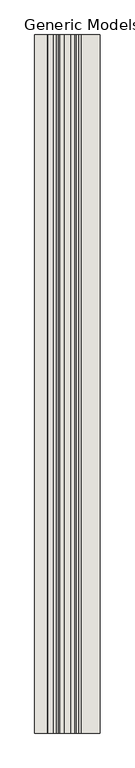
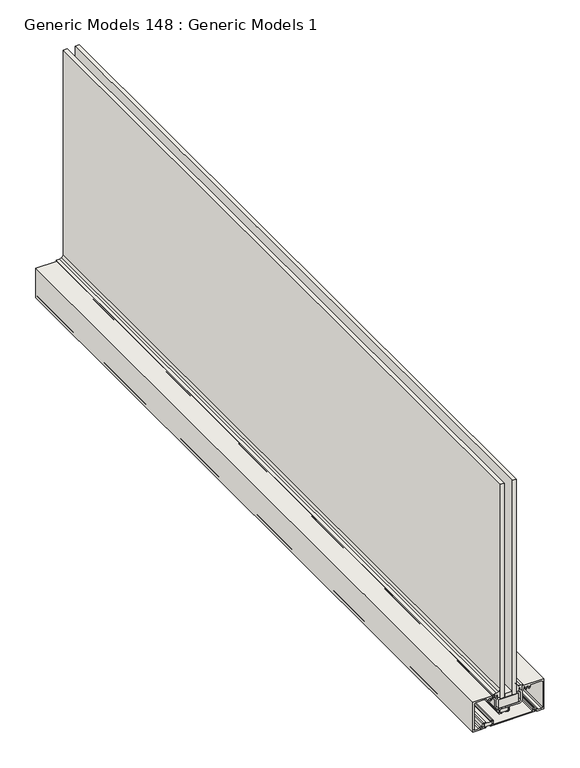
"""IFC4 building model written with IfcOpenShell, lengths in millimetres: wall geometry, Generic Models 148 : Generic Models 1."""

import ifcopenshell
import ifcopenshell.guid

model = None  # the IFC model being written
_history = None  # IfcOwnerHistory: only IFC2X3 demands one
_inside = {}  # id of a spatial element -> (the spatial element, [elements in it])
_under = {}  # id of a project, library or spatial element -> (it, [spatial elements below it])
_declared = {}  # id of a project -> (the project, [libraries it declares])
_typed = {}  # id of a type object -> (the type object, [elements of that type])
_made_of = {}  # id of a material, layer set ... -> (it, [elements and type objects made of it])


def new_model(schema):
    """Start an empty IFC model of exactly this schema.

    Asked for "IFC4X3", IfcOpenShell would pick the latest addendum, in which some entities
    have other attributes; the version numbers below select the first issue.
    IFC2X3 requires an IfcOwnerHistory on every rooted entity: one is made here for all.
    """
    global model, _history
    if schema == "IFC4X3":
        model = ifcopenshell.file(schema_version=(4, 3, 0, 0))
    else:
        model = ifcopenshell.file(schema=schema)
    _inside.clear()
    _under.clear()
    _declared.clear()
    _typed.clear()
    _made_of.clear()
    _history = None
    if model.schema == "IFC2X3":
        org = make("IfcOrganization", Name="unknown")
        user = make(
            "IfcPersonAndOrganization",
            ThePerson=make("IfcPerson", FamilyName="unknown"),
            TheOrganization=org,
        )
        app = make(
            "IfcApplication",
            ApplicationDeveloper=org,
            Version="unknown",
            ApplicationFullName="unknown",
            ApplicationIdentifier="unknown",
        )
        _history = make(
            "IfcOwnerHistory",
            OwningUser=user,
            OwningApplication=app,
            ChangeAction="ADDED",
            CreationDate=0,
        )
    return model


def make(cls, **values):
    """One entity of the class cls with the attributes given. An attribute that is None is left unset."""
    return model.create_entity(
        cls, **{name: value for name, value in values.items() if value is not None}
    )


def rooted(cls, **values):
    """An entity with a GlobalId (a new one), such as an element, a storey or a relation."""
    return make(cls, GlobalId=ifcopenshell.guid.new(), OwnerHistory=_history, **values)


def si_unit(unit_type, name, prefix=None):
    """IfcSIUnit, for example si_unit("LENGTHUNIT", "METRE", prefix="MILLI")."""
    return make("IfcSIUnit", UnitType=unit_type, Prefix=prefix, Name=name)


def assignment(units):
    """IfcUnitAssignment: the units of a project."""
    return None if units is None else make("IfcUnitAssignment", Units=units)


def point(xyz):
    """IfcCartesianPoint."""
    return None if xyz is None else make("IfcCartesianPoint", Coordinates=xyz)


def direction(xyz):
    """IfcDirection."""
    return None if xyz is None else make("IfcDirection", DirectionRatios=xyz)


def frame(location, z_axis=None, x_axis=None):
    """IfcAxis2Placement3D, a coordinate frame: its origin and axes. An axis left out is left unset."""
    return make(
        "IfcAxis2Placement3D",
        Location=point(location),
        Axis=direction(z_axis),
        RefDirection=direction(x_axis),
    )


def frame_2d(location, x_axis=None):
    """IfcAxis2Placement2D, a coordinate frame in the plane: its origin and x axis."""
    return make(
        "IfcAxis2Placement2D", Location=point(location), RefDirection=direction(x_axis)
    )


def origin():
    """The frame at (0, 0, 0) with its axes left unset."""
    return frame((0.0, 0.0, 0.0))


def place(relative_to, where):
    """IfcLocalPlacement: puts the frame where relative to a parent placement (None: the world)."""
    return make(
        "IfcLocalPlacement", PlacementRelTo=relative_to, RelativePlacement=where
    )


def context(
    kind, dimensions, precision=None, world=None, true_north=None, identifier=None
):
    """IfcGeometricRepresentationContext, for example the 3D "Model" context."""
    return make(
        "IfcGeometricRepresentationContext",
        ContextIdentifier=identifier,
        ContextType=kind,
        CoordinateSpaceDimension=dimensions,
        Precision=precision,
        WorldCoordinateSystem=world,
        TrueNorth=true_north,
    )


def project(units=None, contexts=None):
    """IfcProject with its units and contexts."""
    return rooted(
        "IfcProject",
        Name="project",
        RepresentationContexts=contexts,
        UnitsInContext=assignment(units),
    )


def spatial(cls, under=None, at=None, **own):
    """A site, building, storey or space (cls), placed at a placement, below another one or the project."""
    s = rooted(cls, ObjectPlacement=at, **own)
    if under is not None:
        _under.setdefault(under.id(), (under, []))[1].append(s)
    return s


def polyline(points):
    """IfcPolyline through the points."""
    return make("IfcPolyline", Points=[point(p) for p in points])


def circle_curve(where, radius):
    """IfcCircle in the frame where."""
    return make("IfcCircle", Position=where, Radius=radius)


def trimmed(basis, trim1, trim2, sense, master):
    """IfcTrimmedCurve: the piece of a basis curve between two trims."""
    return make(
        "IfcTrimmedCurve",
        BasisCurve=basis,
        Trim1=trim1,
        Trim2=trim2,
        SenseAgreement=sense,
        MasterRepresentation=master,
    )


def segment(curve, same_sense, transition):
    """IfcCompositeCurveSegment."""
    return make(
        "IfcCompositeCurveSegment",
        Transition=transition,
        SameSense=same_sense,
        ParentCurve=curve,
    )


def composite_curve(segments, self_intersect=None):
    """IfcCompositeCurve: segments joined end to end."""
    return make("IfcCompositeCurve", Segments=segments, SelfIntersect=self_intersect)


def outline(outer, holes=None, kind="AREA"):
    """IfcArbitraryClosedProfileDef: a profile drawn as a closed curve; with holes, ...WithVoids."""
    if holes is None:
        return make("IfcArbitraryClosedProfileDef", ProfileType=kind, OuterCurve=outer)
    return make(
        "IfcArbitraryProfileDefWithVoids",
        ProfileType=kind,
        OuterCurve=outer,
        InnerCurves=holes,
    )


def extrude(swept, where, along, depth):
    """IfcExtrudedAreaSolid: the profile swept, set in the frame where, extruded along a direction by depth."""
    return make(
        "IfcExtrudedAreaSolid",
        SweptArea=swept,
        Position=where,
        ExtrudedDirection=direction(along),
        Depth=depth,
    )


def shape(context_of_items, identifier, shape_type, items):
    """IfcShapeRepresentation: the items that make up one representation, for example the "Body"."""
    return make(
        "IfcShapeRepresentation",
        ContextOfItems=context_of_items,
        RepresentationIdentifier=identifier,
        RepresentationType=shape_type,
        Items=items,
    )


def source(mapping_origin, context_of_items, identifier, shape_type, items):
    """IfcRepresentationMap: a shape defined once, which mapped items show again and again."""
    return make(
        "IfcRepresentationMap",
        MappingOrigin=mapping_origin,
        MappedRepresentation=shape(context_of_items, identifier, shape_type, items),
    )


def transform(
    local_origin,
    x_axis=None,
    y_axis=None,
    z_axis=None,
    scale=None,
    scale2=None,
    scale3=None,
    uniform=True,
):
    """IfcCartesianTransformationOperator3D, or its non-uniform kind. x_axis, y_axis, z_axis: its Axis1, 2, 3."""
    if uniform:
        return make(
            "IfcCartesianTransformationOperator3D",
            Axis1=direction(x_axis),
            Axis2=direction(y_axis),
            LocalOrigin=point(local_origin),
            Scale=scale,
            Axis3=direction(z_axis),
        )
    return make(
        "IfcCartesianTransformationOperator3DnonUniform",
        Axis1=direction(x_axis),
        Axis2=direction(y_axis),
        LocalOrigin=point(local_origin),
        Scale=scale,
        Axis3=direction(z_axis),
        Scale2=scale2,
        Scale3=scale3,
    )


def mapped(mapping_source, mapping_target):
    """IfcMappedItem: shows the shape of a source again, moved by a transform."""
    return make(
        "IfcMappedItem", MappingSource=mapping_source, MappingTarget=mapping_target
    )


def made_of(thing, what):
    """Note that an element or type object is made of a material, layer set ...; save() writes the relation."""
    if what is not None:
        _made_of.setdefault(what.id(), (what, []))[1].append(thing)
    return thing


def element(
    cls,
    number,
    at=None,
    inside=None,
    cuts=None,
    type_object=None,
    material=None,
    context=None,
    identifier="Body",
    shape_type=None,
    held_by="IfcProductDefinitionShape",
    body=None,
    shapes=None,
    **own,
):
    """One element of the class cls, such as IfcWall. Its Tag is "e" and its number.

    at: its placement. inside: the storey or other place that contains it. cuts: it is an
    opening in that element (IfcRelVoidsElement). A single representation is given by context,
    identifier, shape_type and body (its items); several are given by shapes. held_by: the class
    of the entity that holds the representations. save() writes the other relations.
    """
    e = rooted(cls, Tag="e%d" % number, ObjectPlacement=at, **own)
    if body is not None:
        shapes = [shape(context, identifier, shape_type, body)]
    if shapes is not None:
        e.Representation = make(held_by, Representations=shapes)
    if inside is not None:
        _inside.setdefault(inside.id(), (inside, []))[1].append(e)
    if cuts is not None:
        rooted(
            "IfcRelVoidsElement", RelatingBuildingElement=cuts, RelatedOpeningElement=e
        )
    if type_object is not None:
        _typed.setdefault(type_object.id(), (type_object, []))[1].append(e)
    return made_of(e, material)


def aggregate(whole, parts):
    """IfcRelAggregates: a whole, such as a stair, and the parts it consists of."""
    return rooted("IfcRelAggregates", RelatingObject=whole, RelatedObjects=parts)


def save(model, path):
    """Write the relations noted so far, then the file.

    IfcRelAggregates (storeys below a building ...), IfcRelContainedInSpatialStructure (elements
    in a storey), IfcRelDefinesByType, IfcRelAssociatesMaterial and IfcRelDeclares: one each for
    every whole, place, type object, material and project.
    """
    for whole, parts in _under.values():
        aggregate(whole, parts)
    for where, things in _inside.values():
        rooted(
            "IfcRelContainedInSpatialStructure",
            RelatedElements=things,
            RelatingStructure=where,
        )
    for kind, things in _typed.values():
        rooted("IfcRelDefinesByType", RelatedObjects=things, RelatingType=kind)
    for what, things in _made_of.values():
        rooted("IfcRelAssociatesMaterial", RelatedObjects=things, RelatingMaterial=what)
    for by, libraries in _declared.values():
        rooted("IfcRelDeclares", RelatingContext=by, RelatedDefinitions=libraries)
    model.write(path)


def generic_models_148_generic_models_1_015d61f0(model_context):
    return source(origin(), model_context, "Body", "SweptSolid", [
        extrude(outline(composite_curve([segment(trimmed(circle_curve(frame_2d((14.097, 50917.5916343)), 1.5795625), [point((15.6765625, 50917.5916343))], [point((14.6380548, 50916.1076271))], False, "CARTESIAN"), True, "CONTINUOUS"), segment(polyline([(14.6380548, 50916.1076271), (10.7648375, 50914.6954892), (10.7648375, 50916.1851634), (8.1835625, 50916.1851634), (8.1835625, 50911.8671634), (6.5484375, 50911.8671634), (6.5484375, 50921.1478154), (8.1835625, 50921.1478154), (8.1835625, 50917.5664154), (14.8034375, 50917.5664154), (14.8034375, 50921.1478154), (15.6765625, 50921.1478154), (15.6765625, 50917.5916343)]), True, "CONTINUOUS")], self_intersect=False)), frame((0.0, 0.0, 0.0), z_axis=(0.0, 1.0, 0.0), x_axis=(0.0, 0.0, 1.0)), (0.0, 0.0, 1.0), 1219.2),
        extrude(outline(composite_curve([segment(trimmed(circle_curve(frame_2d((12.446, 50996.7010997)), 0.7064375), [point((12.6878975, 50997.3648312))], [point((11.740864, 50996.6582372))], True, "CARTESIAN"), True, "CONTINUOUS"), segment(polyline([(11.740864, 50996.6582372), (8.1835625, 50996.6582372), (8.1835625, 50933.5636529)]), True, "CONTINUOUS"), segment(trimmed(circle_curve(frame_2d((8.89, 50933.5636529)), 0.7064375), [point((8.1835625, 50933.5636529))], [point((8.89, 50932.8572154))], True, "CARTESIAN"), True, "CONTINUOUS"), segment(polyline([(8.89, 50932.8572154), (14.097, 50932.8572154)]), True, "CONTINUOUS"), segment(trimmed(circle_curve(frame_2d((14.097, 50931.2776529)), 1.5795625), [point((14.097, 50932.8572154))], [point((15.6765625, 50931.2776529))], False, "CARTESIAN"), True, "CONTINUOUS"), segment(polyline([(15.6765625, 50931.2776529), (15.6765625, 50927.8946904), (14.8034375, 50927.8946904), (14.8034375, 50931.4760904), (8.1835625, 50931.4760904), (8.1835625, 50927.8946904), (6.5484375, 50927.8946904), (6.5484375, 51002.3573622), (8.1835625, 51002.3573622), (8.1835625, 50998.0393622), (10.7648375, 50998.0393622), (10.7648375, 50999.5290364), (16.009985, 50997.616706)]), True, "CONTINUOUS"), segment(trimmed(circle_curve(frame_2d((15.7734, 50996.9677997)), 0.6906895), [point((16.009985, 50997.616706))], [point((15.5374141, 50996.3186752))], False, "CARTESIAN"), True, "CONTINUOUS"), segment(polyline([(15.5374141, 50996.3186752), (12.6878975, 50997.3648312)]), True, "CONTINUOUS")], self_intersect=False)), frame((0.0, 0.0, 0.0), z_axis=(0.0, 1.0, 0.0), x_axis=(0.0, 0.0, 1.0)), (0.0, 0.0, 1.0), 1219.2),
        extrude(outline(composite_curve([segment(trimmed(circle_curve(frame_2d((34.29, 50974.625)), 2.54), [point((34.29, 50977.165))], [point((31.75, 50974.625))], True, "CARTESIAN"), True, "CONTINUOUS"), segment(polyline([(31.75, 50974.625), (31.75, 50953.1493), (29.718, 50953.1493), (29.718, 50956.7307), (23.495, 50956.7307), (23.495, 50953.1493), (22.225, 50953.1493), (22.225, 50956.7307)]), True, "CONTINUOUS"), segment(trimmed(circle_curve(frame_2d((24.003, 50956.7307)), 1.778), [point((22.225, 50956.7307))], [point((24.003, 50958.5087))], False, "CARTESIAN"), True, "CONTINUOUS"), segment(polyline([(24.003, 50958.5087), (29.21, 50958.5087)]), True, "CONTINUOUS"), segment(trimmed(circle_curve(frame_2d((29.21, 50959.0167)), 0.508), [point((29.21, 50958.5087))], [point((29.718, 50959.0167))], True, "CARTESIAN"), True, "CONTINUOUS"), segment(polyline([(29.718, 50959.0167), (29.718, 50974.879)]), True, "CONTINUOUS"), segment(trimmed(circle_curve(frame_2d((34.036, 50974.879)), 4.318), [point((29.718, 50974.879))], [point((34.036, 50979.197))], False, "CARTESIAN"), True, "CONTINUOUS"), segment(polyline([(34.036, 50979.197), (49.1342256, 50979.197), (50.8386835, 50980.9028737)]), True, "CONTINUOUS"), segment(trimmed(circle_curve(frame_2d((52.7253201, 50979.017803)), 2.667), [point((50.8386835, 50980.9028737))], [point((52.7253201, 50981.684803))], False, "CARTESIAN"), True, "CONTINUOUS"), segment(polyline([(52.7253201, 50981.684803), (54.61, 50981.684803)]), True, "CONTINUOUS"), segment(trimmed(circle_curve(frame_2d((54.61, 50982.192803)), 0.508), [point((54.61, 50981.684803))], [point((55.118, 50982.192803))], True, "CARTESIAN"), True, "CONTINUOUS"), segment(polyline([(55.118, 50982.192803), (55.118, 50984.0043351)]), True, "CONTINUOUS"), segment(trimmed(circle_curve(frame_2d((54.61, 50984.0043351)), 0.508), [point((55.118, 50984.0043351))], [point((54.3683568, 50984.4511825))], True, "CARTESIAN"), True, "CONTINUOUS"), segment(trimmed(circle_curve(frame_2d((52.3748, 50988.137673)), 4.191), [point((54.3683568, 50984.4511825))], [point((49.3268, 50985.2611861))], False, "CARTESIAN"), True, "CONTINUOUS"), segment(polyline([(49.3268, 50985.2611861), (49.3268, 50986.3779094), (50.2850807, 50986.931173)]), True, "CONTINUOUS"), segment(trimmed(circle_curve(frame_2d((52.3748, 50988.137673)), 2.413), [point((50.2850807, 50986.931173))], [point((50.2850807, 50989.344173))], True, "CARTESIAN"), True, "CONTINUOUS"), segment(polyline([(50.2850807, 50989.344173), (49.3268, 50989.8974366), (49.3268, 50991.0141599)]), True, "CONTINUOUS"), segment(trimmed(circle_curve(frame_2d((52.3748, 50988.137673)), 4.191), [point((49.3268, 50991.0141599))], [point((54.3683568, 50991.8241635))], False, "CARTESIAN"), True, "CONTINUOUS"), segment(trimmed(circle_curve(frame_2d((54.61, 50992.2710109)), 0.508), [point((54.3683568, 50991.8241635))], [point((55.118, 50992.2710109))], True, "CARTESIAN"), True, "CONTINUOUS"), segment(polyline([(55.118, 50992.2710109), (55.118, 51010.756373)]), True, "CONTINUOUS"), segment(trimmed(circle_curve(frame_2d((53.594, 51010.756373)), 1.524), [point((55.118, 51010.756373))], [point((53.594, 51012.280373))], True, "CARTESIAN"), True, "CONTINUOUS"), segment(polyline([(53.594, 51012.280373), (9.906, 51012.280373)]), True, "CONTINUOUS"), segment(trimmed(circle_curve(frame_2d((9.906, 51010.756373)), 1.524), [point((9.906, 51012.280373))], [point((8.382, 51010.756373))], True, "CARTESIAN"), True, "CONTINUOUS"), segment(polyline([(8.382, 51010.756373), (8.382, 51004.700214)]), True, "CONTINUOUS"), segment(trimmed(circle_curve(frame_2d((8.89, 51003.263373)), 1.524), [point((8.382, 51004.700214))], [point((10.414, 51003.263373))], False, "CARTESIAN"), True, "CONTINUOUS"), segment(polyline([(10.414, 51003.263373), (10.414, 50998.5052015)]), True, "CONTINUOUS"), segment(trimmed(circle_curve(frame_2d((9.9568, 51000.012173)), 1.5748), [point((10.414, 50998.5052015))], [point((8.382, 51000.012173))], False, "CARTESIAN"), True, "CONTINUOUS"), segment(polyline([(8.382, 51000.012173), (8.382, 51002.755373), (6.35, 51002.755373), (6.35, 51014.312373), (57.15, 51014.312373), (57.15, 50979.652803), (52.46214, 50979.652803), (50.5841, 50977.773203), (50.5841, 50976.2991491), (53.5813, 50975.640873), (55.3593, 50975.640873), (55.3593, 50974.624873), (49.3141, 50974.624873), (49.3141, 50976.657)]), True, "CONTINUOUS"), segment(trimmed(circle_curve(frame_2d((48.8061, 50976.657)), 0.508), [point((49.3141, 50976.657))], [point((48.8061, 50977.165))], True, "CARTESIAN"), True, "CONTINUOUS"), segment(polyline([(48.8061, 50977.165), (34.29, 50977.165)]), True, "CONTINUOUS")], self_intersect=False)), frame((0.0, 0.0, 0.0), z_axis=(0.0, 1.0, 0.0), x_axis=(0.0, 0.0, 1.0)), (0.0, 0.0, 1.0), 1219.2),
        extrude(outline(composite_curve([segment(trimmed(circle_curve(frame_2d((48.8061, 50937.667873)), 0.508), [point((48.8061, 50937.159873))], [point((49.3141, 50937.667873))], True, "CARTESIAN"), True, "CONTINUOUS"), segment(polyline([(49.3141, 50937.667873), (49.3141, 50939.7), (55.3593, 50939.7), (55.3593, 50938.684), (53.5813, 50938.684), (50.5841, 50938.0257239), (50.5841, 50936.55167), (52.46214, 50934.67207), (57.15, 50934.67207), (57.15, 50900.0125), (6.35, 50900.0125), (6.35, 50911.5695), (8.382, 50911.5695), (8.382, 50914.3127)]), True, "CONTINUOUS"), segment(trimmed(circle_curve(frame_2d((9.9568, 50914.3127)), 1.5748), [point((8.382, 50914.3127))], [point((10.414, 50915.8196715))], False, "CARTESIAN"), True, "CONTINUOUS"), segment(polyline([(10.414, 50915.8196715), (10.414, 50911.0615)]), True, "CONTINUOUS"), segment(trimmed(circle_curve(frame_2d((8.89, 50911.0615)), 1.524), [point((10.414, 50911.0615))], [point((8.382, 50909.624659))], False, "CARTESIAN"), True, "CONTINUOUS"), segment(polyline([(8.382, 50909.624659), (8.382, 50903.568373)]), True, "CONTINUOUS"), segment(trimmed(circle_curve(frame_2d((9.906, 50903.568373)), 1.524), [point((8.382, 50903.568373))], [point((9.906, 50902.044373))], True, "CARTESIAN"), True, "CONTINUOUS"), segment(polyline([(9.906, 50902.044373), (53.594, 50902.044373)]), True, "CONTINUOUS"), segment(trimmed(circle_curve(frame_2d((53.594, 50903.568373)), 1.524), [point((53.594, 50902.044373))], [point((55.118, 50903.568373))], True, "CARTESIAN"), True, "CONTINUOUS"), segment(polyline([(55.118, 50903.568373), (55.118, 50922.0538621)]), True, "CONTINUOUS"), segment(trimmed(circle_curve(frame_2d((54.61, 50922.0538621)), 0.508), [point((55.118, 50922.0538621))], [point((54.3683568, 50922.5007095))], True, "CARTESIAN"), True, "CONTINUOUS"), segment(trimmed(circle_curve(frame_2d((52.3748, 50926.1872)), 4.191), [point((54.3683568, 50922.5007095))], [point((49.3268, 50923.3107131))], False, "CARTESIAN"), True, "CONTINUOUS"), segment(polyline([(49.3268, 50923.3107131), (49.3268, 50924.4274364), (50.2850807, 50924.9807)]), True, "CONTINUOUS"), segment(trimmed(circle_curve(frame_2d((52.3748, 50926.1872)), 2.413), [point((50.2850807, 50924.9807))], [point((50.2850807, 50927.3937))], True, "CARTESIAN"), True, "CONTINUOUS"), segment(polyline([(50.2850807, 50927.3937), (49.3268, 50927.9469636), (49.3268, 50929.0636869)]), True, "CONTINUOUS"), segment(trimmed(circle_curve(frame_2d((52.3748, 50926.1872)), 4.191), [point((49.3268, 50929.0636869))], [point((54.3683568, 50929.8736905))], False, "CARTESIAN"), True, "CONTINUOUS"), segment(trimmed(circle_curve(frame_2d((54.61, 50930.3205379)), 0.508), [point((54.3683568, 50929.8736905))], [point((55.118, 50930.3205379))], True, "CARTESIAN"), True, "CONTINUOUS"), segment(polyline([(55.118, 50930.3205379), (55.118, 50932.13207)]), True, "CONTINUOUS"), segment(trimmed(circle_curve(frame_2d((54.61, 50932.13207)), 0.508), [point((55.118, 50932.13207))], [point((54.61, 50932.64007))], True, "CARTESIAN"), True, "CONTINUOUS"), segment(polyline([(54.61, 50932.64007), (52.7253201, 50932.64007)]), True, "CONTINUOUS"), segment(trimmed(circle_curve(frame_2d((52.7253201, 50935.30707)), 2.667), [point((52.7253201, 50932.64007))], [point((50.8386835, 50933.4219993))], False, "CARTESIAN"), True, "CONTINUOUS"), segment(polyline([(50.8386835, 50933.4219993), (49.1342256, 50935.127873), (34.036, 50935.127873)]), True, "CONTINUOUS"), segment(trimmed(circle_curve(frame_2d((34.036, 50939.445873)), 4.318), [point((34.036, 50935.127873))], [point((29.718, 50939.445873))], False, "CARTESIAN"), True, "CONTINUOUS"), segment(polyline([(29.718, 50939.445873), (29.718, 50941.439773), (24.003, 50941.439773)]), True, "CONTINUOUS"), segment(trimmed(circle_curve(frame_2d((24.003, 50943.217773)), 1.778), [point((24.003, 50941.439773))], [point((22.225, 50943.217773))], False, "CARTESIAN"), True, "CONTINUOUS"), segment(polyline([(22.225, 50943.217773), (22.225, 50946.7993), (23.495, 50946.7993), (23.495, 50943.2179), (29.718, 50943.2179), (29.718, 50946.7993), (31.75, 50946.7993), (31.75, 50939.699873)]), True, "CONTINUOUS"), segment(trimmed(circle_curve(frame_2d((34.29, 50939.699873)), 2.54), [point((31.75, 50939.699873))], [point((34.29, 50937.159873))], True, "CARTESIAN"), True, "CONTINUOUS"), segment(polyline([(34.29, 50937.159873), (48.8061, 50937.159873)]), True, "CONTINUOUS")], self_intersect=False)), frame((0.0, 0.0, 0.0), z_axis=(0.0, 1.0, 0.0), x_axis=(0.0, 0.0, 1.0)), (0.0, 0.0, 1.0), 1219.2),
        extrude(outline(polyline([(50973.0629678, 0.0), (50941.7098428, 0.0), (50941.7098428, 1219.2), (50973.0629678, 1219.2), (50973.0629678, 0.0)])), frame((0.0, 0.0, 32.5992301), z_axis=(0.0, 0.0, 1.0), x_axis=(1.0, 0.0, 0.0)), (0.0, 0.0, 1.0), 14.684375),
        extrude(outline(polyline([(50950.82359, 0.0), (50944.47359, 0.0), (50944.47359, 1219.2), (50950.82359, 1219.2), (50950.82359, 0.0)])), frame((0.0, 0.0, 47.625), z_axis=(0.0, 0.0, 1.0), x_axis=(1.0, 0.0, 0.0)), (0.0, 0.0, 1.0), 365.125),
        extrude(outline(polyline([(50969.87359, 0.0), (50963.52359, 0.0), (50963.52359, 1219.2), (50969.87359, 1219.2), (50969.87359, 0.0)])), frame((0.0, 0.0, 47.625), z_axis=(0.0, 0.0, 1.0), x_axis=(1.0, 0.0, 0.0)), (0.0, 0.0, 1.0), 365.125),
        extrude(outline(polyline([(50963.3251525, 0.0), (50951.0220275, 0.0), (50951.0220275, 1219.2), (50963.3251525, 1219.2), (50963.3251525, 0.0)])), frame((0.0, 0.0, 47.625), z_axis=(0.0, 0.0, 1.0), x_axis=(1.0, 0.0, 0.0)), (0.0, 0.0, 1.0), 6.35),
        extrude(outline(composite_curve([segment(trimmed(circle_curve(frame_2d((64.2304882, 50976.1426745)), 4.9643345), [point((59.3077698, 50976.7841265))], [point((60.6315489, 50972.7232808))], True, "CARTESIAN"), True, "CONTINUOUS"), segment(polyline([(60.6315489, 50972.7232808), (63.5908154, 50970.1744071), (50.679329, 50970.1744071), (50.679329, 50974.1558571), (56.1304866, 50974.1558571), (56.1304866, 50975.8945302), (54.2354153, 50975.8945302), (51.2348926, 50976.553536), (51.2348926, 50977.5441268), (52.8805452, 50979.1911463), (57.5342084, 50979.1911463), (57.5342084, 50980.9684916), (58.6865882, 50980.9684916)]), True, "CONTINUOUS"), segment(trimmed(circle_curve(frame_2d((47.3152777, 50977.1420956)), 11.9978335), [point((58.6865882, 50980.9684916))], [point((59.3077698, 50976.7841265))], False, "CARTESIAN"), True, "CONTINUOUS")], self_intersect=False)), frame((0.0, 0.0, 0.0), z_axis=(0.0, 1.0, 0.0), x_axis=(0.0, 0.0, 1.0)), (0.0, 0.0, 1.0), 1219.2),
        extrude(outline(composite_curve([segment(trimmed(circle_curve(frame_2d((47.3152777, 50937.0578364)), 11.9978335), [point((59.3077698, 50937.4158055))], [point((58.6865882, 50933.2314404))], False, "CARTESIAN"), True, "CONTINUOUS"), segment(polyline([(58.6865882, 50933.2314404), (57.5342084, 50933.2314404), (57.5342084, 50935.0087857), (52.8805452, 50935.0087857), (51.2348926, 50936.6558052), (51.2348926, 50937.646396), (54.2354153, 50938.3054018), (56.1304866, 50938.3054018), (56.1304866, 50940.0440749), (50.679329, 50940.0440749), (50.679329, 50944.0255249), (63.5908154, 50944.0255249), (60.6315489, 50941.4766512)]), True, "CONTINUOUS"), segment(trimmed(circle_curve(frame_2d((64.2304882, 50938.0572575)), 4.9643345), [point((60.6315489, 50941.4766512))], [point((59.3077698, 50937.4158055))], True, "CARTESIAN"), True, "CONTINUOUS")], self_intersect=False)), frame((0.0, 0.0, 0.0), z_axis=(0.0, 1.0, 0.0), x_axis=(0.0, 0.0, 1.0)), (0.0, 0.0, 1.0), 1219.2),
        extrude(outline(polyline([(50931.0792154, 0.0), (50917.9632904, 0.0), (50917.9632904, 1219.2), (50931.0792154, 1219.2), (50931.0792154, 0.0)])), frame((0.0, 0.0, 8.5804375), z_axis=(0.0, 0.0, 1.0), x_axis=(1.0, 0.0, 0.0)), (0.0, 0.0, 1.0), 5.826125),
        extrude(outline(polyline([(50956.5322625, 0.0), (50943.4163375, 0.0), (50943.4163375, 1219.2), (50956.5322625, 1219.2), (50956.5322625, 0.0)])), frame((0.0, 0.0, 23.6934375), z_axis=(0.0, 0.0, 1.0), x_axis=(1.0, 0.0, 0.0)), (0.0, 0.0, 1.0), 5.826125),
    ])


if __name__ == "__main__":
    model = new_model("IFC4")
    model_context = context("Model", 3, world=origin())
    ifc_project = project(units=[si_unit("LENGTHUNIT", "METRE", prefix="MILLI")], contexts=[model_context])
    site = spatial("IfcSite", under=ifc_project)
    building = spatial("IfcBuilding", under=site)
    placement = place(None, origin())
    generic_models_148_generic_models_1_shape = generic_models_148_generic_models_1_015d61f0(model_context)
    element("IfcWall", 1, ObjectType="Generic Models 148 : Generic Models 1", at=placement, inside=building, context=model_context, shape_type="MappedRepresentation", body=[
        mapped(generic_models_148_generic_models_1_shape, transform((0.0, 0.0, 0.0), x_axis=(1.0, 0.0, 0.0), y_axis=(0.0, 1.0, 0.0), z_axis=(0.0, 0.0, 1.0))),
    ])
    save(model, "model.ifc")

# Revit data of these elements
# Element 1 (IfcWall, "Generic Models 148 : Generic Models 1")
#   Materials on its faces: "ALUM. STOREFRONT W/ INSULATED GLAZING"
# Materials
#   "ALUM. STOREFRONT W/ INSULATED GLAZING": class "Glass", colour RGB 196 205 210, transparency 0.85, Description = "Soda Lime Glass", Cost = 0
